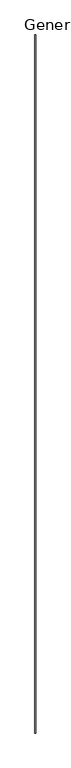
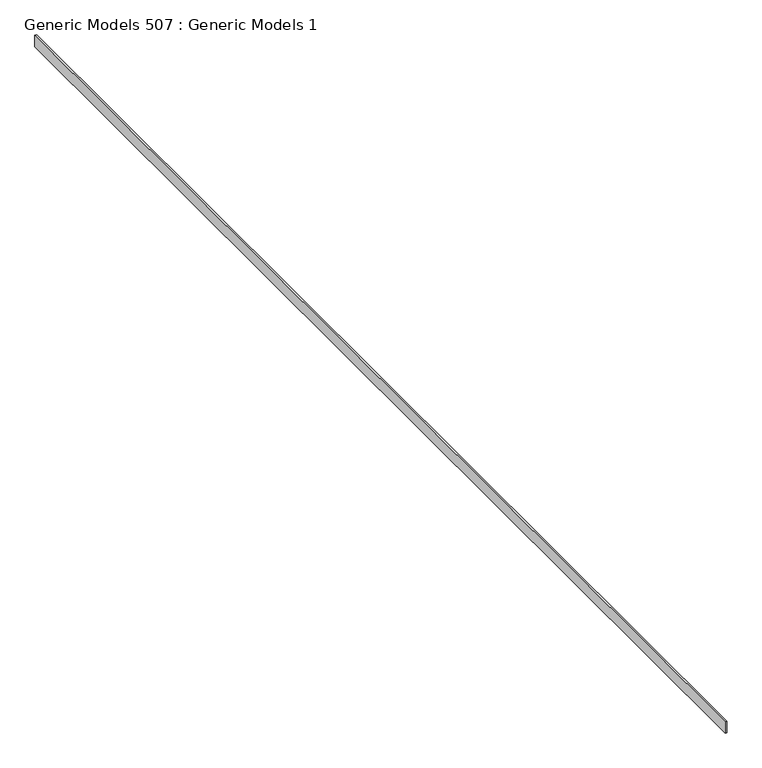
"""IFC4 building model written with IfcOpenShell, lengths in millimetres: proxy geometry, Generic Models 507 : Generic Models 1."""

from ifc_helpers import new_model, si_unit, frame, origin, place, context, project, spatial, polyline, outline, extrude, source, transform, mapped, element, save


def generic_models_507_generic_models_1_37fa60e8(model_context):
    return source(origin(), model_context, "Body", "SweptSolid", [
        extrude(outline(polyline([(8517.4383294, 551.8769662), (8528.5508294, 551.8769662), (8528.5508294, -7068.1230338), (8517.4383294, -7068.1230338), (8517.4383294, 551.8769662)])), frame((0.0, 0.0, 126214.8150364), z_axis=(0.0, 0.0, 1.0), x_axis=(1.0, 0.0, 0.0)), (0.0, 0.0, 1.0), 76.2),
    ])


if __name__ == "__main__":
    model = new_model("IFC4")
    model_context = context("Model", 3, world=origin())
    ifc_project = project(units=[si_unit("LENGTHUNIT", "METRE", prefix="MILLI")], contexts=[model_context])
    site = spatial("IfcSite", under=ifc_project)
    building = spatial("IfcBuilding", under=site)
    placement = place(None, origin())
    generic_models_507_generic_models_1_shape = generic_models_507_generic_models_1_37fa60e8(model_context)
    element("IfcBuildingElementProxy", 1, Name="Generic Models 507 : Generic Models 1", ObjectType="Generic Models 507 : Generic Models 1", at=placement, inside=building, context=model_context, shape_type="MappedRepresentation", body=[
        mapped(generic_models_507_generic_models_1_shape, transform((0.0, 0.0, 0.0), x_axis=(1.0, 0.0, 0.0), y_axis=(0.0, 1.0, 0.0), z_axis=(0.0, 0.0, 1.0))),
    ])
    save(model, "model.ifc")

# Revit data of these elements
# Element 1 (IfcBuildingElementProxy, "Generic Models 507 : Generic Models 1")
#   Materials on its faces: "_SIDING VENT - COR-A-VENT - 7/16\" X 3\""
# Materials
#   "_SIDING VENT - COR-A-VENT - 7/16\" X 3\"": class "Generic", colour RGB 190 220 196, transparency 0, Cost = 0
